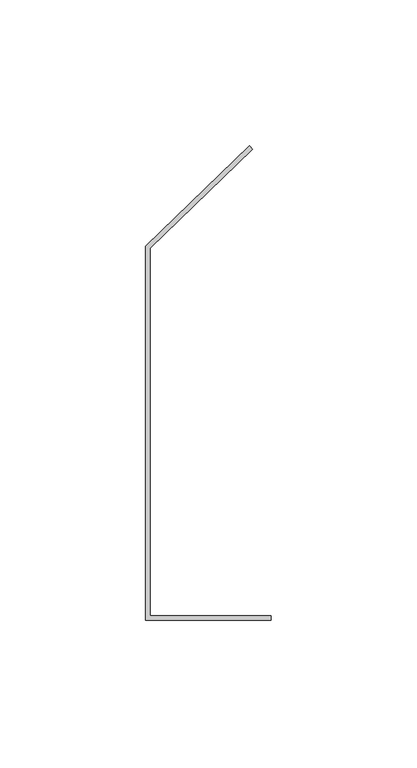
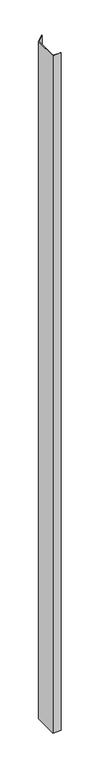
"""IFC4 building model written with IfcOpenShell, lengths in millimetres: proxy geometry, Generic Models 11:Generic Models 1:306267:Generic Models 1:306267 : Generic Models 11:Generic Models 1:306267:300405:Generic Models 1:306267:Generic Models 1:306267 : Generic Models 11:Generic Models 1:306267:300405 : Generic Models 11:Generic Models 1:306267:Generic Models 1:306267 : Generic Models 11:Generic Models 1:306267:300405:22 : Generic Models 11:Generic Models 1:306267:Generic Models 1:306267 : Generic Models 11:Generic Models 1:306267:300405:Generic Models 1:306267:Generic Models 1:306267 : Generic Models 11:Generic Models 1:306267:300405 : Generic Models 11:Generic Models 1:306267:Generic Models 1:306267 : Generic Models 11:Generic Models 1:306267:300405:300182."""

from ifc_helpers import new_model, si_unit, frame, origin, place, context, project, spatial, polyline, outline, extrude, source, transform, mapped, element, save


def generic_models_bb0783e2(model_context):
    return source(origin(), model_context, "Body", "SweptSolid", [
        extrude(outline(polyline([(578579.828326, -568277.8386667), (578579.828326, -568149.6454795), (578615.3859082, -568115.1783298), (578616.5085764, -568116.3009979), (578581.415826, -568150.3175706), (578581.415826, -568276.2511667), (578622.8845989, -568276.2511667), (578622.8845989, -568277.8386667), (578579.828326, -568277.8386667)])), frame((0.0, 0.0, 4853.797603), z_axis=(0.0, 0.0, 1.0), x_axis=(1.0, 0.0, 0.0)), (0.0, 0.0, 1.0), 3695.7),
    ])


if __name__ == "__main__":
    model = new_model("IFC4")
    model_context = context("Model", 3, world=origin())
    ifc_project = project(units=[si_unit("LENGTHUNIT", "METRE", prefix="MILLI")], contexts=[model_context])
    site = spatial("IfcSite", under=ifc_project)
    building = spatial("IfcBuilding", under=site)
    placement = place(None, origin())
    generic_models_shape = generic_models_bb0783e2(model_context)
    element("IfcBuildingElementProxy", 1, Name="Generic Models 11:Generic Models 1:306267:Generic Models 1:306267 : Generic Models 11:Generic Models 1:306267:300405:Generic Models 1:306267:Generic Models 1:306267 : Generic Models 11:Generic Models 1:306267:300405 : Generic Models 11:Generic Models 1:306267:Generic Models 1:306267 : Generic Models 11:Generic Models 1:306267:300405:22 : Generic Models 11:Generic Models 1:306267:Generic Models 1:306267 : Generic Models 11:Generic Models 1:306267:300405:Generic Models 1:306267:Generic Models 1:306267 : Generic Models 11:Generic Models 1:306267:300405 : Generic Models 11:Generic Models 1:306267:Generic Models 1:306267 : Generic Models 11:Generic Models 1:306267:300405:300182", ObjectType="Generic Models 11:Generic Models 1:306267:Generic Models 1:306267 : Generic Models 11:Generic Models 1:306267:300405:Generic Models 1:306267:Generic Models 1:306267 : Generic Models 11:Generic Models 1:306267:300405 : Generic Models 11:Generic Models 1:306267:Generic Models 1:306267 : Generic Models 11:Generic Models 1:306267:300405:22 : Generic Models 11:Generic Models 1:306267:Generic Models 1:306267 : Generic Models 11:Generic Models 1:306267:300405:Generic Models 1:306267:Generic Models 1:306267 : Generic Models 11:Generic Models 1:306267:300405 : Generic Models 11:Generic Models 1:306267:Generic Models 1:306267 : Generic Models 11:Generic Models 1:306267:300405:300182", at=placement, inside=building, context=model_context, shape_type="MappedRepresentation", body=[
        mapped(generic_models_shape, transform((0.0, 0.0, 0.0), x_axis=(1.0, 0.0, 0.0), y_axis=(0.0, 1.0, 0.0), z_axis=(0.0, 0.0, 1.0))),
    ])
    save(model, "model.ifc")

# Revit data of these elements
# Type "Generic Models 11:Generic Models 1:306267:Generic Models 1:306267 : Generic Models 11:Generic Models 1:306267:300405:Generic Models 1:306267:Generic Models 1:306267 : Generic Models 11:Generic Models 1:306267:300405 : Generic Models 11:Generic Models 1:306267:Generic Models 1:306267 : Generic Models 11:Generic Models 1:306267:300405:22 : Generic Models 11:Generic Models 1:306267:Generic Models 1:306267 : Generic Models 11:Generic Models 1:306267:300405:Generic Models 1:306267:Generic Models 1:306267 : Generic Models 11:Generic Models 1:306267:300405 : Generic Models 11:Generic Models 1:306267:Generic Models 1:306267 : Generic Models 11:Generic Models 1:306267:300405:300182"
#   NameOverride = "Generic Models 11:Generic Models 1:306267:Generic Models 1:306267 : Generic Models 11:Generic Models 1:306267:300405:Generic Models 1:306267:Generic Models 1:306267 : Generic Models 11:Generic Models 1:306267:300405 : Generic Models 11:Generic Models 1:306267:Generic Models 1:306267 : Generic Models 11:Generic Models 1:306267:300405:300182"
#   ObjectTypeOverride = "Generic Models 1:306267:Generic Models 1:306267 : Generic Models 11:Generic Models 1:306267:300405 : Generic Models 11:Generic Models 1:306267:Generic Models 1:306267 : Generic Models 11:Generic Models 1:306267:300405"
#   Reference = "Generic Models 1"
#   Tag = "300182"
# Element 1 (IfcBuildingElementProxy, "Generic Models 11:Generic Models 1:306267:Generic Models 1:306267 : Generic Models 11:Generic Models 1:306267:300405:Generic Models 1:306267:Generic Models 1:306267 : Generic Models 11:Generic Models 1:306267:300405 : Generic Models 11:Generic Models 1:306267:Generic Models 1:306267 : Generic Models 11:Generic Models 1:306267:300405:22 : Generic Models 11:Generic Models 1:306267:Generic Models 1:306267 : Generic Models 11:Generic Models 1:306267:300405:Generic Models 1:306267:Generic Models 1:306267 : Generic Models 11:Generic Models 1:306267:300405 : Generic Models 11:Generic Models 1:306267:Generic Models 1:306267 : Generic Models 11:Generic Models 1:306267:300405:300182")
#   Materials on its faces: "BRAKE METAL CLOSURE TRIM"
# Materials
#   "BRAKE METAL CLOSURE TRIM": class "Unassigned", colour RGB 210 209 208, transparency 0, Cost = 0
